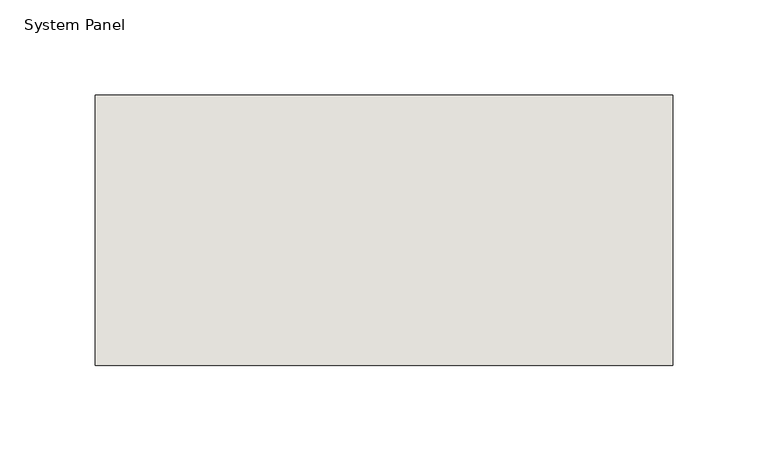
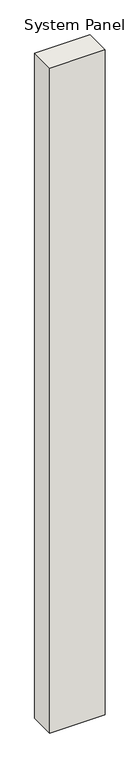
"""IFC4 building model written with IfcOpenShell, lengths in millimetres: wall geometry, System Panel : NLRS_21_CWP_hsb-vulling minerale wol 142 _gen_rsf."""

from ifc_helpers import new_model, si_unit, origin, origin_with_axes, place, context, project, spatial, polyline, outline, extrude, source, transform, mapped, element, save


def system_panel_d3f78fb4(model_context):
    return source(origin(), model_context, "Body", "SweptSolid", [
        extrude(outline(polyline([(151.4999998, -71.0), (-151.4999998, -71.0), (-151.4999998, 71.0), (151.4999998, 71.0), (151.4999998, -71.0)])), origin_with_axes(), (0.0, 0.0, 1.0), 3849.0),
    ])


if __name__ == "__main__":
    model = new_model("IFC4")
    model_context = context("Model", 3, world=origin())
    ifc_project = project(units=[si_unit("LENGTHUNIT", "METRE", prefix="MILLI")], contexts=[model_context])
    site = spatial("IfcSite", under=ifc_project)
    building = spatial("IfcBuilding", under=site)
    placement = place(None, origin())
    system_panel_shape = system_panel_d3f78fb4(model_context)
    element("IfcWall", 1, ObjectType="System Panel : NLRS_21_CWP_hsb-vulling minerale wol 142 _gen_rsf", at=placement, inside=building, context=model_context, shape_type="MappedRepresentation", body=[
        mapped(system_panel_shape, transform((0.0, 0.0, 0.0), x_axis=(1.0, 0.0, 0.0), y_axis=(0.0, 1.0, 0.0), z_axis=(0.0, 0.0, 1.0))),
    ])
    save(model, "model.ifc")

# Revit data of these elements
# Type "System Panel : NLRS_21_CWP_hsb-vulling minerale wol 142 _gen_rsf"
#   Type IfcGUID = "07M7mRoiH1CR8m_RSKIwpC"
#   Assembly Code = "21.23"
#   IfcExportAs = "IfcWall"
# Element 1 (IfcWall, "System Panel : NLRS_21_CWP_hsb-vulling minerale wol 142 _gen_rsf")
#   Materials on its faces: "NLRS_m1_isolatie minerale wol_gen_rsf"
# Materials
#   "NLRS_m1_isolatie minerale wol_gen_rsf": class "M - Anorganische materialen", colour RGB 200 200 140, transparency 0, Keynote = "m1", Manufacturer = "Revit Standards Foundation", URL = "www.revitstandards.org", Description = "isolatie minerale wol", Cost = 0
